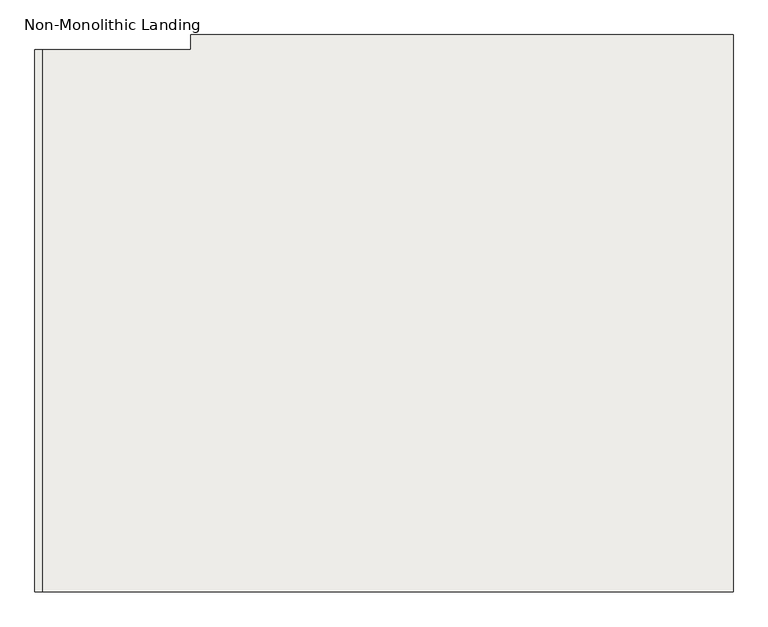
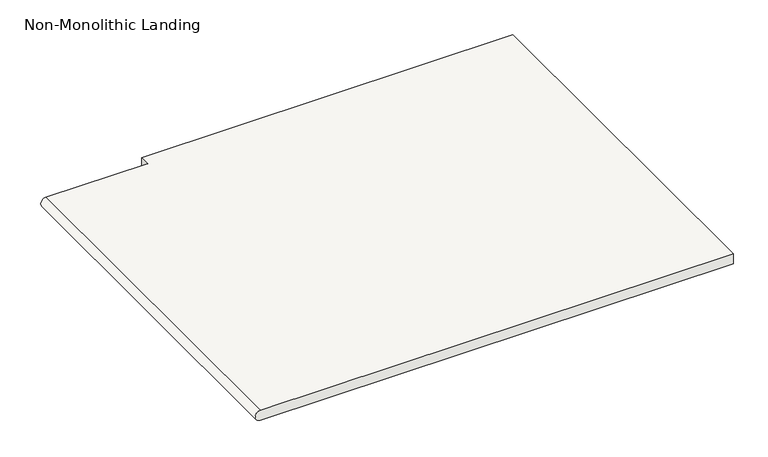
"""IFC4 building model written with IfcOpenShell, lengths in millimetres: slab geometry, Non-Monolithic Landing."""

import ifcopenshell
import ifcopenshell.guid

model = None  # the IFC model being written
_history = None  # IfcOwnerHistory: only IFC2X3 demands one
_inside = {}  # id of a spatial element -> (the spatial element, [elements in it])
_under = {}  # id of a project, library or spatial element -> (it, [spatial elements below it])
_declared = {}  # id of a project -> (the project, [libraries it declares])
_typed = {}  # id of a type object -> (the type object, [elements of that type])
_made_of = {}  # id of a material, layer set ... -> (it, [elements and type objects made of it])


def new_model(schema):
    """Start an empty IFC model of exactly this schema.

    Asked for "IFC4X3", IfcOpenShell would pick the latest addendum, in which some entities
    have other attributes; the version numbers below select the first issue.
    IFC2X3 requires an IfcOwnerHistory on every rooted entity: one is made here for all.
    """
    global model, _history
    if schema == "IFC4X3":
        model = ifcopenshell.file(schema_version=(4, 3, 0, 0))
    else:
        model = ifcopenshell.file(schema=schema)
    _inside.clear()
    _under.clear()
    _declared.clear()
    _typed.clear()
    _made_of.clear()
    _history = None
    if model.schema == "IFC2X3":
        org = make("IfcOrganization", Name="unknown")
        user = make(
            "IfcPersonAndOrganization",
            ThePerson=make("IfcPerson", FamilyName="unknown"),
            TheOrganization=org,
        )
        app = make(
            "IfcApplication",
            ApplicationDeveloper=org,
            Version="unknown",
            ApplicationFullName="unknown",
            ApplicationIdentifier="unknown",
        )
        _history = make(
            "IfcOwnerHistory",
            OwningUser=user,
            OwningApplication=app,
            ChangeAction="ADDED",
            CreationDate=0,
        )
    return model


def make(cls, **values):
    """One entity of the class cls with the attributes given. An attribute that is None is left unset."""
    return model.create_entity(
        cls, **{name: value for name, value in values.items() if value is not None}
    )


def rooted(cls, **values):
    """An entity with a GlobalId (a new one), such as an element, a storey or a relation."""
    return make(cls, GlobalId=ifcopenshell.guid.new(), OwnerHistory=_history, **values)


def si_unit(unit_type, name, prefix=None):
    """IfcSIUnit, for example si_unit("LENGTHUNIT", "METRE", prefix="MILLI")."""
    return make("IfcSIUnit", UnitType=unit_type, Prefix=prefix, Name=name)


def assignment(units):
    """IfcUnitAssignment: the units of a project."""
    return None if units is None else make("IfcUnitAssignment", Units=units)


def point(xyz):
    """IfcCartesianPoint."""
    return None if xyz is None else make("IfcCartesianPoint", Coordinates=xyz)


def direction(xyz):
    """IfcDirection."""
    return None if xyz is None else make("IfcDirection", DirectionRatios=xyz)


def frame(location, z_axis=None, x_axis=None):
    """IfcAxis2Placement3D, a coordinate frame: its origin and axes. An axis left out is left unset."""
    return make(
        "IfcAxis2Placement3D",
        Location=point(location),
        Axis=direction(z_axis),
        RefDirection=direction(x_axis),
    )


def origin():
    """The frame at (0, 0, 0) with its axes left unset."""
    return frame((0.0, 0.0, 0.0))


def place(relative_to, where):
    """IfcLocalPlacement: puts the frame where relative to a parent placement (None: the world)."""
    return make(
        "IfcLocalPlacement", PlacementRelTo=relative_to, RelativePlacement=where
    )


def context(
    kind, dimensions, precision=None, world=None, true_north=None, identifier=None
):
    """IfcGeometricRepresentationContext, for example the 3D "Model" context."""
    return make(
        "IfcGeometricRepresentationContext",
        ContextIdentifier=identifier,
        ContextType=kind,
        CoordinateSpaceDimension=dimensions,
        Precision=precision,
        WorldCoordinateSystem=world,
        TrueNorth=true_north,
    )


def project(units=None, contexts=None):
    """IfcProject with its units and contexts."""
    return rooted(
        "IfcProject",
        Name="project",
        RepresentationContexts=contexts,
        UnitsInContext=assignment(units),
    )


def spatial(cls, under=None, at=None, **own):
    """A site, building, storey or space (cls), placed at a placement, below another one or the project."""
    s = rooted(cls, ObjectPlacement=at, **own)
    if under is not None:
        _under.setdefault(under.id(), (under, []))[1].append(s)
    return s


def circle_curve(where, radius):
    """IfcCircle in the frame where."""
    return make("IfcCircle", Position=where, Radius=radius)


def shape(context_of_items, identifier, shape_type, items):
    """IfcShapeRepresentation: the items that make up one representation, for example the "Body"."""
    return make(
        "IfcShapeRepresentation",
        ContextOfItems=context_of_items,
        RepresentationIdentifier=identifier,
        RepresentationType=shape_type,
        Items=items,
    )


def source(mapping_origin, context_of_items, identifier, shape_type, items):
    """IfcRepresentationMap: a shape defined once, which mapped items show again and again."""
    return make(
        "IfcRepresentationMap",
        MappingOrigin=mapping_origin,
        MappedRepresentation=shape(context_of_items, identifier, shape_type, items),
    )


def transform(
    local_origin,
    x_axis=None,
    y_axis=None,
    z_axis=None,
    scale=None,
    scale2=None,
    scale3=None,
    uniform=True,
):
    """IfcCartesianTransformationOperator3D, or its non-uniform kind. x_axis, y_axis, z_axis: its Axis1, 2, 3."""
    if uniform:
        return make(
            "IfcCartesianTransformationOperator3D",
            Axis1=direction(x_axis),
            Axis2=direction(y_axis),
            LocalOrigin=point(local_origin),
            Scale=scale,
            Axis3=direction(z_axis),
        )
    return make(
        "IfcCartesianTransformationOperator3DnonUniform",
        Axis1=direction(x_axis),
        Axis2=direction(y_axis),
        LocalOrigin=point(local_origin),
        Scale=scale,
        Axis3=direction(z_axis),
        Scale2=scale2,
        Scale3=scale3,
    )


def mapped(mapping_source, mapping_target):
    """IfcMappedItem: shows the shape of a source again, moved by a transform."""
    return make(
        "IfcMappedItem", MappingSource=mapping_source, MappingTarget=mapping_target
    )


def made_of(thing, what):
    """Note that an element or type object is made of a material, layer set ...; save() writes the relation."""
    if what is not None:
        _made_of.setdefault(what.id(), (what, []))[1].append(thing)
    return thing


def element(
    cls,
    number,
    at=None,
    inside=None,
    cuts=None,
    type_object=None,
    material=None,
    context=None,
    identifier="Body",
    shape_type=None,
    held_by="IfcProductDefinitionShape",
    body=None,
    shapes=None,
    **own,
):
    """One element of the class cls, such as IfcWall. Its Tag is "e" and its number.

    at: its placement. inside: the storey or other place that contains it. cuts: it is an
    opening in that element (IfcRelVoidsElement). A single representation is given by context,
    identifier, shape_type and body (its items); several are given by shapes. held_by: the class
    of the entity that holds the representations. save() writes the other relations.
    """
    e = rooted(cls, Tag="e%d" % number, ObjectPlacement=at, **own)
    if body is not None:
        shapes = [shape(context, identifier, shape_type, body)]
    if shapes is not None:
        e.Representation = make(held_by, Representations=shapes)
    if inside is not None:
        _inside.setdefault(inside.id(), (inside, []))[1].append(e)
    if cuts is not None:
        rooted(
            "IfcRelVoidsElement", RelatingBuildingElement=cuts, RelatedOpeningElement=e
        )
    if type_object is not None:
        _typed.setdefault(type_object.id(), (type_object, []))[1].append(e)
    return made_of(e, material)


def aggregate(whole, parts):
    """IfcRelAggregates: a whole, such as a stair, and the parts it consists of."""
    return rooted("IfcRelAggregates", RelatingObject=whole, RelatedObjects=parts)


def save(model, path):
    """Write the relations noted so far, then the file.

    IfcRelAggregates (storeys below a building ...), IfcRelContainedInSpatialStructure (elements
    in a storey), IfcRelDefinesByType, IfcRelAssociatesMaterial and IfcRelDeclares: one each for
    every whole, place, type object, material and project.
    """
    for whole, parts in _under.values():
        aggregate(whole, parts)
    for where, things in _inside.values():
        rooted(
            "IfcRelContainedInSpatialStructure",
            RelatedElements=things,
            RelatingStructure=where,
        )
    for kind, things in _typed.values():
        rooted("IfcRelDefinesByType", RelatedObjects=things, RelatingType=kind)
    for what, things in _made_of.values():
        rooted("IfcRelAssociatesMaterial", RelatedObjects=things, RelatingMaterial=what)
    for by, libraries in _declared.values():
        rooted("IfcRelDeclares", RelatingContext=by, RelatedDefinitions=libraries)
    model.write(path)


def plane_surface(at):
    """IfcPlane: the flat surface through the origin of the frame at, square to its z axis."""
    return make("IfcPlane", Position=at)


def cylinder_surface(at, radius):
    """IfcCylindricalSurface: all points at the distance radius from the z axis of the frame at."""
    return make("IfcCylindricalSurface", Position=at, Radius=radius)


def advanced_brep(points, edges, surfaces, faces):
    """IfcAdvancedBrep: a solid bounded by faces that lie on surfaces and meet in shared edges.

    An edge is (start, end): straight between two places in points (the first is 0);
    or (start, end, curve); or (start, end, curve, False) where it runs against its curve.
    A face is (place in surfaces, loops), or (place, loops, False) where it looks against
    its surface's normal. A loop lists edges by number (the first is 1), with a minus sign
    where the edge is run from its end to its start. The first loop is the outer one.
    """
    corners = [point(p) for p in points]
    vertices = [make("IfcVertexPoint", VertexGeometry=c) for c in corners]
    made = []
    for start, end, *more in edges:
        made.append(
            make(
                "IfcEdgeCurve",
                EdgeStart=vertices[start],
                EdgeEnd=vertices[end],
                EdgeGeometry=more[0] if more else make("IfcPolyline", Points=[corners[start], corners[end]]),
                SameSense=more[1] if len(more) > 1 else True,
            )
        )
    hull = []
    for where, loops, *sense in faces:
        bounds = []
        for j, loop in enumerate(loops):
            ring = [make("IfcOrientedEdge", EdgeElement=made[abs(k) - 1], Orientation=k > 0) for k in loop]
            bounds.append(
                make(
                    "IfcFaceOuterBound" if j == 0 else "IfcFaceBound",
                    Bound=make("IfcEdgeLoop", EdgeList=ring),
                    Orientation=True,
                )
            )
        hull.append(make("IfcAdvancedFace", Bounds=bounds, FaceSurface=surfaces[where], SameSense=sense[0] if sense else True))
    return make("IfcAdvancedBrep", Outer=make("IfcClosedShell", CfsFaces=hull))


def non_monolithic_landing_3de38245(model_context):
    return source(origin(), model_context, "Body", "AdvancedBrep", [
        advanced_brep(
        [(6239.7741968, -13363.3557429, 1689.1), (6239.7741968, -13363.3557429, 1714.5), (6239.7741968, -12448.9557429, 1714.5), (6239.7741968, -12448.9557429, 1689.1), (7404.2789345, -13363.3557429, 1714.5), (7404.2789345, -12448.9557429, 1714.5), (7404.2789345, -12423.5557429, 1714.5), (6489.8789345, -12423.5557429, 1714.5), (6489.8789345, -12448.9557429, 1714.5), (7404.2789345, -13363.3557429, 1689.1), (6489.8789345, -12448.9557429, 1689.1), (6489.8789345, -12423.5557429, 1689.1), (7404.2789345, -12423.5557429, 1689.1), (7404.2789345, -12448.9557429, 1689.1)],
        [
            (0, 1, circle_curve(frame((6239.7741968, -13363.3557429, 1701.8), z_axis=(0.0, 1.0, 0.0), x_axis=(1.0, 0.0, 0.0)), 12.7)),
            (1, 2),
            (2, 3, circle_curve(frame((6239.7741968, -12448.9557429, 1701.8), z_axis=(0.0, -1.0, 0.0), x_axis=(1.0, 0.0, 0.0)), 12.7)),
            (3, 0),
            (1, 4),
            (4, 5),
            (5, 6),
            (6, 7),
            (7, 8),
            (8, 2),
            (9, 0),
            (3, 10),
            (10, 11),
            (11, 12),
            (12, 13),
            (13, 9),
            (9, 4),
            (13, 5),
            (12, 6),
            (11, 7),
            (10, 8),
        ],
        [
            cylinder_surface(frame((6239.7741968, -13363.3557429, 1701.8), z_axis=(0.0, -1.0, 0.0), x_axis=(1.0, 0.0, 0.0)), 12.7),
            plane_surface(frame((6239.7741968, -12448.9557429, 1714.5), z_axis=(0.0, 0.0, 1.0), x_axis=(0.0, -1.0, 0.0))),
            plane_surface(frame((6239.7741968, -12448.9557429, 1689.1), z_axis=(0.0, 0.0, -1.0), x_axis=(0.0, 1.0, 0.0))),
            plane_surface(frame((6239.7741968, -13363.3557429, 1714.5), z_axis=(0.0, -1.0, 0.0), x_axis=(0.0, 0.0, -1.0))),
            plane_surface(frame((7404.2789345, -13363.3557429, 1714.5), z_axis=(1.0, 0.0, 0.0), x_axis=(0.0, 0.0, -1.0))),
            plane_surface(frame((7404.2789345, -12448.9557429, 1714.5), z_axis=(1.0, 0.0, 0.0), x_axis=(0.0, 0.0, -1.0))),
            plane_surface(frame((7404.2789345, -12423.5557429, 1714.5), z_axis=(0.0, 1.0, 0.0), x_axis=(0.0, 0.0, -1.0))),
            plane_surface(frame((6489.8789345, -12423.5557429, 1714.5), z_axis=(-1.0, 0.0, 0.0), x_axis=(0.0, 0.0, -1.0))),
            plane_surface(frame((6489.8789345, -12448.9557429, 1714.5), z_axis=(0.0, 1.0, 0.0), x_axis=(0.0, 0.0, -1.0))),
        ],
        [
            (0, [[1, 2, 3, 4]]),
            (1, [[5, 6, 7, 8, 9, 10, -2]]),
            (2, [[11, -4, 12, 13, 14, 15, 16]]),
            (3, [[-5, -1, -11, 17]]),
            (4, [[-6, -17, -16, 18]]),
            (5, [[-7, -18, -15, 19]]),
            (6, [[-8, -19, -14, 20]]),
            (7, [[-9, -20, -13, 21]]),
            (8, [[-10, -21, -12, -3]]),
        ],
    ),
    ])


if __name__ == "__main__":
    model = new_model("IFC4")
    model_context = context("Model", 3, world=origin())
    ifc_project = project(units=[si_unit("LENGTHUNIT", "METRE", prefix="MILLI")], contexts=[model_context])
    site = spatial("IfcSite", under=ifc_project)
    building = spatial("IfcBuilding", under=site)
    placement = place(None, origin())
    non_monolithic_landing_shape = non_monolithic_landing_3de38245(model_context)
    element("IfcSlab", 1, ObjectType="Non-Monolithic Landing", at=placement, inside=building, context=model_context, shape_type="MappedRepresentation", body=[
        mapped(non_monolithic_landing_shape, transform((0.0, 0.0, 0.0), x_axis=(1.0, 0.0, 0.0), y_axis=(0.0, 1.0, 0.0), z_axis=(0.0, 0.0, 1.0))),
    ])
    save(model, "model.ifc")

# Revit data of these elements
# Element 1 (IfcSlab, "Non-Monolithic Landing")
#   Materials on its faces: "Cherry"
# Materials
#   "Cherry": class "Wood", colour RGB 233 182 144, transparency 0, Description = "Prunus Serotina", Cost = 0
